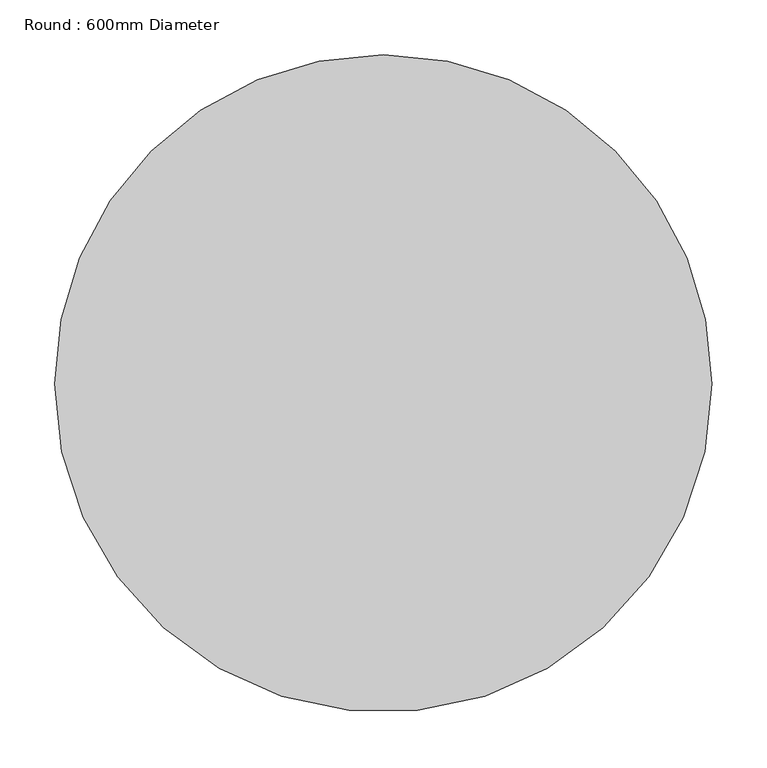
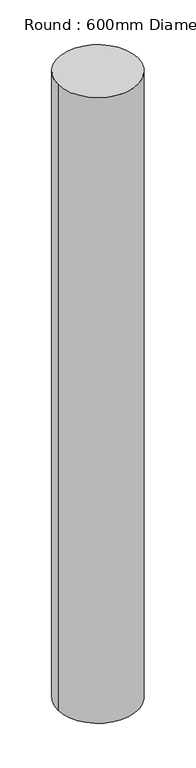
"""IFC4 building model written with IfcOpenShell, lengths in millimetres: column geometry, Round : 600mm Diameter."""

from ifc_helpers import new_model, si_unit, point, frame, origin, origin_2d, place, context, project, spatial, circle_curve, trimmed, segment, composite_curve, outline, extrude, source, transform, mapped, element, save


def round_600mm_diameter_31934321(model_context):
    return source(origin(), model_context, "Body", "SweptSolid", [
        extrude(outline(composite_curve([segment(trimmed(circle_curve(origin_2d(), 300.0), [point((300.0, 0.0))], [point((-300.0, 0.0))], False, "CARTESIAN"), True, "CONTINUOUS"), segment(trimmed(circle_curve(origin_2d(), 300.0), [point((-300.0, 0.0))], [point((0.0, 300.0))], False, "CARTESIAN"), True, "CONTINUOUS"), segment(trimmed(circle_curve(origin_2d(), 300.0), [point((0.0, 300.0))], [point((300.0, 0.0))], False, "CARTESIAN"), True, "CONTINUOUS")], self_intersect=False)), frame((0.0, 0.0, 143170.0), z_axis=(0.0, 0.0, 1.0), x_axis=(1.0, 0.0, 0.0)), (0.0, 0.0, 1.0), 4950.0),
    ])


if __name__ == "__main__":
    model = new_model("IFC4")
    model_context = context("Model", 3, world=origin())
    ifc_project = project(units=[si_unit("LENGTHUNIT", "METRE", prefix="MILLI")], contexts=[model_context])
    site = spatial("IfcSite", under=ifc_project)
    building = spatial("IfcBuilding", under=site)
    placement = place(None, origin())
    round_600mm_diameter_shape = round_600mm_diameter_31934321(model_context)
    element("IfcColumn", 1, ObjectType="Round : 600mm Diameter", at=placement, inside=building, context=model_context, shape_type="MappedRepresentation", body=[
        mapped(round_600mm_diameter_shape, transform((0.0, 0.0, 0.0), x_axis=(1.0, 0.0, 0.0), y_axis=(0.0, 1.0, 0.0), z_axis=(0.0, 0.0, 1.0))),
    ])
    save(model, "model.ifc")

# Revit data of these elements
# Type "Round : 600mm Diameter"
#   Keynote = "G"
#   Diameter = 600.00 mm
#   Offset Base = 0.00 mm
#   Offset Top = 0.00 mm
#   built-in parameter 1002110 = 8421504
#   built-in parameter 1002106 = element 3
#   Material = Concrete - Cast In Situ
# Element 1 (IfcColumn, "Round : 600mm Diameter")
#   Materials on its faces: "Concrete - Cast In Situ"
# Materials
#   "Concrete - Cast In Situ": class "Unassigned", colour RGB 255 255 255, transparency 0, Keynote = "E10/132", Cost = 0
